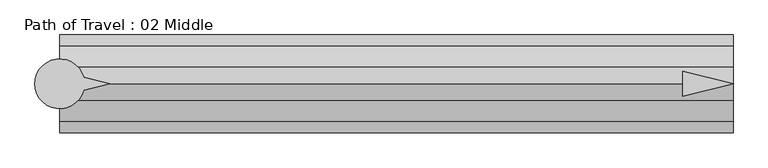
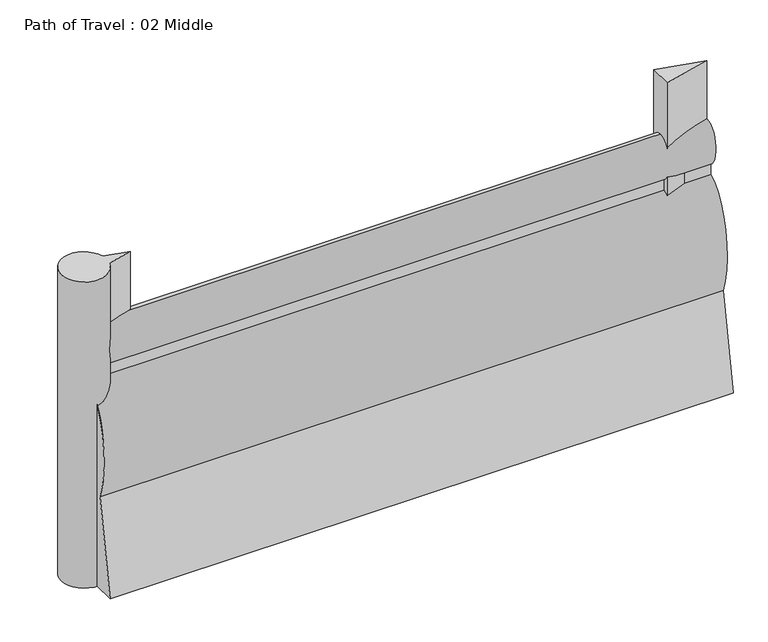
"""IFC4 building model written with IfcOpenShell, lengths in millimetres: proxy geometry, Path of Travel : 02 Middle."""

from ifc_helpers import new_model, si_unit, point, frame, frame_2d, origin, origin_with_axes, place, context, project, spatial, polyline, circle_curve, ellipse_curve, trimmed, segment, composite_curve, outline, extrude, source, transform, mapped, element, save
from ifc_brep_helpers import plane_surface, extruded_surface, advanced_brep


def path_of_travel_02_middle_6add304d(model_context):
    return source(origin(), model_context, "Body", "SolidModel", [
        advanced_brep(
        [(227.5554837, 0.0, 1727.2), (227.5554837, 42.9018657, 1436.6534209), (227.5554837, 42.9018657, 1363.4763406), (227.5554837, 184.1186263, 643.4144547), (227.5554837, 297.5699544, 0.0), (227.5554837, 145.6574193, 0.0), (227.5554837, 0.0, 584.2), (227.5554837, -145.6574193, 0.0), (227.5554837, -297.5699544, 0.0), (227.5554837, -184.1186263, 643.4144547), (227.5554837, -42.9018657, 1363.4763406), (227.5554837, -42.9018657, 1436.6534209), (4323.3079095, 0.0, 1727.2), (4323.3079095, -42.9018657, 1436.6534209), (4323.3079095, -42.9018657, 1363.4763406), (4323.3079095, -184.1186263, 643.4144547), (4323.3079095, -297.5699544, 0.0), (4323.3079095, -145.6574193, 0.0), (4323.3079095, 0.0, 584.2), (4323.3079095, 145.6574193, 0.0), (4323.3079095, 297.5699544, 0.0), (4323.3079095, 184.1186263, 643.4144547), (4323.3079095, 42.9018657, 1363.4763406), (4323.3079095, 42.9018657, 1436.6534209)],
        [
            (0, 1, ellipse_curve(frame((227.5554837, 0.0, 1574.8), z_axis=(-1.0, 0.0, 0.0), x_axis=(0.0, 0.0, 1.0)), 152.4, 101.6)),
            (1, 2),
            (2, 3, ellipse_curve(frame((227.5554837, 0.0, 914.4), z_axis=(-1.0, 0.0, 0.0), x_axis=(0.0, 0.0, -1.0)), 457.2, 228.6)),
            (3, 4),
            (4, 5),
            (5, 6),
            (6, 7),
            (7, 8),
            (8, 9),
            (9, 10, ellipse_curve(frame((227.5554837, 0.0, 914.4), z_axis=(-1.0, 0.0, 0.0), x_axis=(0.0, 0.0, -1.0)), 457.2, 228.6)),
            (10, 11),
            (11, 0, ellipse_curve(frame((227.5554837, 0.0, 1574.8), z_axis=(-1.0, 0.0, 0.0), x_axis=(0.0, 0.0, 1.0)), 152.4, 101.6)),
            (12, 13, ellipse_curve(frame((4323.3079095, 0.0, 1574.8), z_axis=(1.0, 0.0, 0.0), x_axis=(0.0, 0.0, 1.0)), 152.4, 101.6)),
            (13, 14),
            (14, 15, ellipse_curve(frame((4323.3079095, 0.0, 914.4), z_axis=(1.0, 0.0, 0.0), x_axis=(0.0, 0.0, -1.0)), 457.2, 228.6)),
            (15, 16),
            (16, 17),
            (17, 18),
            (18, 19),
            (19, 20),
            (20, 21),
            (21, 22, ellipse_curve(frame((4323.3079095, 0.0, 914.4), z_axis=(1.0, 0.0, 0.0), x_axis=(0.0, 0.0, -1.0)), 457.2, 228.6)),
            (22, 23),
            (23, 12, ellipse_curve(frame((4323.3079095, 0.0, 1574.8), z_axis=(1.0, 0.0, 0.0), x_axis=(0.0, 0.0, 1.0)), 152.4, 101.6)),
            (0, 12),
            (23, 1),
            (22, 2),
            (21, 3),
            (20, 4),
            (19, 5),
            (18, 6),
            (17, 7),
            (16, 8),
            (15, 9),
            (14, 10),
            (13, 11),
        ],
        [
            plane_surface(frame((227.5554837, 0.0, 0.0), z_axis=(-1.0, 0.0, 0.0), x_axis=(0.0, 0.0, 1.0))),
            plane_surface(frame((4323.3079095, 0.0, 0.0), z_axis=(1.0, 0.0, 0.0), x_axis=(0.0, 0.0, 1.0))),
            extruded_surface(trimmed(ellipse_curve(frame((4323.3079095, 0.0, 1574.8), z_axis=(-1.0, 0.0, 0.0), x_axis=(0.0, 0.0, 1.0)), 152.4, 101.6), [point((4323.3079095, 0.0, 1727.2))], [point((4323.3079095, 42.9018657, 1436.6534209))], True, "CARTESIAN"), (-4095.7524258000003, 0.0, 0.0), 4095.7524258000003),
            plane_surface(frame((227.5554837, 42.9018657, 1436.6534209), z_axis=(0.0, 1.0, 0.0), x_axis=(1.0, 0.0, 0.0))),
            extruded_surface(trimmed(ellipse_curve(frame((4323.3079095, 0.0, 914.4), z_axis=(-1.0, 0.0, 0.0), x_axis=(0.0, 0.0, -1.0)), 457.2, 228.6), [point((4323.3079095, 42.9018657, 1363.4763406))], [point((4323.3079095, 184.1186263, 643.4144547))], True, "CARTESIAN"), (-4095.7524258000003, 0.0, 0.0), 4095.7524258000003),
            plane_surface(frame((227.5554837, 184.1186263, 643.4144547), z_axis=(0.0, 0.9848077530122078, 0.1736481776669322), x_axis=(1.0, 0.0, 0.0))),
            plane_surface(frame((227.5554837, 297.5699544, 0.0), z_axis=(0.0, 0.0, -1.0), x_axis=(1.0, 0.0, 0.0))),
            plane_surface(frame((227.5554837, 145.6574193, 0.0), z_axis=(0.0, -0.9702957262760199, -0.2419218955995739), x_axis=(1.0, 0.0, 0.0))),
            plane_surface(frame((227.5554837, 0.0, 584.2), z_axis=(0.0, 0.9702957262759961, -0.24192189559966923), x_axis=(1.0, 0.0, 0.0))),
            plane_surface(frame((227.5554837, -145.6574193, 0.0), z_axis=(0.0, 0.0, -1.0), x_axis=(1.0, 0.0, 0.0))),
            plane_surface(frame((227.5554837, -297.5699544, 0.0), z_axis=(0.0, -0.984807753012208, 0.17364817766693066), x_axis=(1.0, 0.0, 0.0))),
            extruded_surface(trimmed(ellipse_curve(frame((4323.3079095, 0.0, 914.4), z_axis=(-1.0, 0.0, 0.0), x_axis=(0.0, 0.0, -1.0)), 457.2, 228.6), [point((4323.3079095, -184.1186263, 643.4144547))], [point((4323.3079095, -42.9018657, 1363.4763406))], True, "CARTESIAN"), (-4095.7524258000003, 0.0, 0.0), 4095.7524258000003),
            plane_surface(frame((227.5554837, -42.9018657, 1363.4763406), z_axis=(0.0, -1.0, 0.0), x_axis=(1.0, 0.0, 0.0))),
            extruded_surface(trimmed(ellipse_curve(frame((4323.3079095, 0.0, 1574.8), z_axis=(-1.0, 0.0, 0.0), x_axis=(0.0, 0.0, 1.0)), 152.4, 101.6), [point((4323.3079095, -42.9018657, 1436.6534209))], [point((4323.3079095, 0.0, 1727.2))], True, "CARTESIAN"), (-4095.7524258000003, 0.0, 0.0), 4095.7524258000003),
        ],
        [
            (0, [[1, 2, 3, 4, 5, 6, 7, 8, 9, 10, 11, 12]]),
            (1, [[13, 14, 15, 16, 17, 18, 19, 20, 21, 22, 23, 24]]),
            (2, [[-1, 25, -24, 26]]),
            (3, [[-2, -26, -23, 27]]),
            (4, [[-3, -27, -22, 28]]),
            (5, [[-4, -28, -21, 29]]),
            (6, [[-5, -29, -20, 30]]),
            (7, [[-6, -30, -19, 31]]),
            (8, [[-7, -31, -18, 32]]),
            (9, [[-8, -32, -17, 33]]),
            (10, [[-9, -33, -16, 34]]),
            (11, [[-10, -34, -15, 35]]),
            (12, [[-11, -35, -14, 36]]),
            (13, [[-12, -36, -13, -25]]),
        ],
    ),
        extrude(outline(polyline([(4017.3027629, 76.2006338), (4323.3079095, 0.0), (4017.3027629, -76.2006338), (4017.3027629, 76.2006338)])), origin_with_axes(), (0.0, 0.0, 1.0), 2129.5973753),
        extrude(outline(composite_curve([segment(polyline([(372.7837828, 39.4440225), (531.182385, 0.0), (372.7837828, -39.4440225)]), True, "CONTINUOUS"), segment(trimmed(circle_curve(frame_2d((227.2200886, 0.0)), 150.8131956), [point((372.7837828, -39.4440225))], [point((372.7837828, 39.4440225))], False, "CARTESIAN"), True, "CONTINUOUS")], self_intersect=False)), origin_with_axes(), (0.0, 0.0, 1.0), 2129.5973753),
    ])


if __name__ == "__main__":
    model = new_model("IFC4")
    model_context = context("Model", 3, world=origin())
    ifc_project = project(units=[si_unit("LENGTHUNIT", "METRE", prefix="MILLI")], contexts=[model_context])
    site = spatial("IfcSite", under=ifc_project)
    building = spatial("IfcBuilding", under=site)
    placement = place(None, origin())
    path_of_travel_02_middle_shape = path_of_travel_02_middle_6add304d(model_context)
    element("IfcBuildingElementProxy", 1, Name="Path of Travel : 02 Middle", ObjectType="Path of Travel : 02 Middle", at=placement, inside=building, context=model_context, shape_type="MappedRepresentation", body=[
        mapped(path_of_travel_02_middle_shape, transform((0.0, 0.0, 0.0), x_axis=(1.0, 0.0, 0.0), y_axis=(0.0, 1.0, 0.0), z_axis=(0.0, 0.0, 1.0))),
    ])
    save(model, "model.ifc")

# Revit data of these elements
# Type "Path of Travel : 02 Middle"
#   Path of Egress [instance default] = 4' - 0"
#   built-in parameter 1001306 [instance default] = 4 (stored number, unit not read)
#   Dot at Start = no
#   Arrow in Middle = yes
#   Arrow at End = no
#   Egress Path = none
# Element 1 (IfcBuildingElementProxy, "Path of Travel : 02 Middle")
#   Path of Egress = 13' - 5.2501"
#   built-in parameter 1001306 = 13.4375 (stored number, unit not read)
